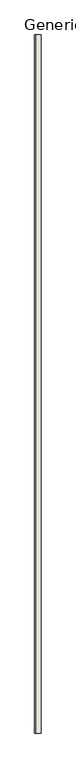
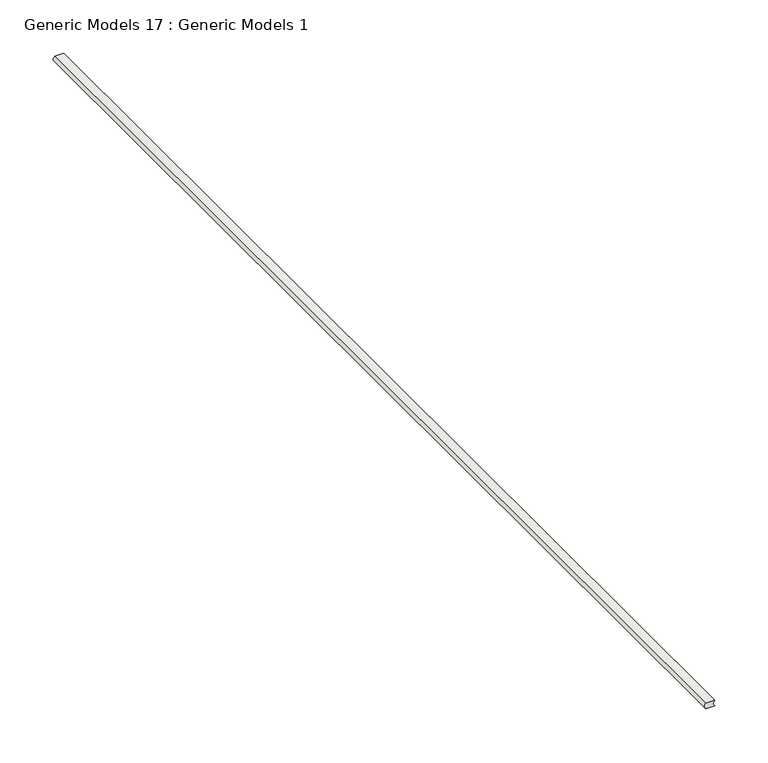
"""IFC4 building model written with IfcOpenShell, lengths in millimetres: wall geometry, Generic Models 17 : Generic Models 1."""

from ifc_helpers import new_model, si_unit, point, frame, frame_2d, origin, place, context, project, spatial, polyline, circle_curve, trimmed, segment, composite_curve, outline, extrude, source, transform, mapped, element, save


def generic_models_17_generic_models_1_2237eccc(model_context):
    return source(origin(), model_context, "Body", "SweptSolid", [
        extrude(outline(composite_curve([segment(trimmed(circle_curve(frame_2d((3.175, 141242.7897405)), 4.3100275), [point((0.0, 141239.875))], [point((6.35, 141239.875))], True, "CARTESIAN"), True, "CONTINUOUS"), segment(polyline([(6.35, 141239.875), (6.35, 141230.35)]), True, "CONTINUOUS"), segment(trimmed(circle_curve(frame_2d((3.175, 141233.2647405)), 4.3100275), [point((6.35, 141230.35))], [point((0.0, 141230.35))], False, "CARTESIAN"), True, "CONTINUOUS"), segment(polyline([(0.0, 141230.35), (0.0, 141239.875)]), True, "CONTINUOUS")], self_intersect=False)), frame((0.0, 0.0, 0.0), z_axis=(0.0, 1.0, 0.0), x_axis=(0.0, 0.0, 1.0)), (0.0, 0.0, 1.0), 1219.2),
    ])


if __name__ == "__main__":
    model = new_model("IFC4")
    model_context = context("Model", 3, world=origin())
    ifc_project = project(units=[si_unit("LENGTHUNIT", "METRE", prefix="MILLI")], contexts=[model_context])
    site = spatial("IfcSite", under=ifc_project)
    building = spatial("IfcBuilding", under=site)
    placement = place(None, origin())
    generic_models_17_generic_models_1_shape = generic_models_17_generic_models_1_2237eccc(model_context)
    element("IfcWall", 1, ObjectType="Generic Models 17 : Generic Models 1", at=placement, inside=building, context=model_context, shape_type="MappedRepresentation", body=[
        mapped(generic_models_17_generic_models_1_shape, transform((0.0, 0.0, 0.0), x_axis=(1.0, 0.0, 0.0), y_axis=(0.0, 1.0, 0.0), z_axis=(0.0, 0.0, 1.0))),
    ])
    save(model, "model.ifc")

# Revit data of these elements
# Element 1 (IfcWall, "Generic Models 17 : Generic Models 1")
#   Materials on its faces: "ACOUSTICAL SEALANT OR FIRE SEALANT, IF RATED WALL"
# Materials
#   "ACOUSTICAL SEALANT OR FIRE SEALANT, IF RATED WALL": class "Unassigned", colour RGB 120 120 120, transparency 0, Cost = 0
